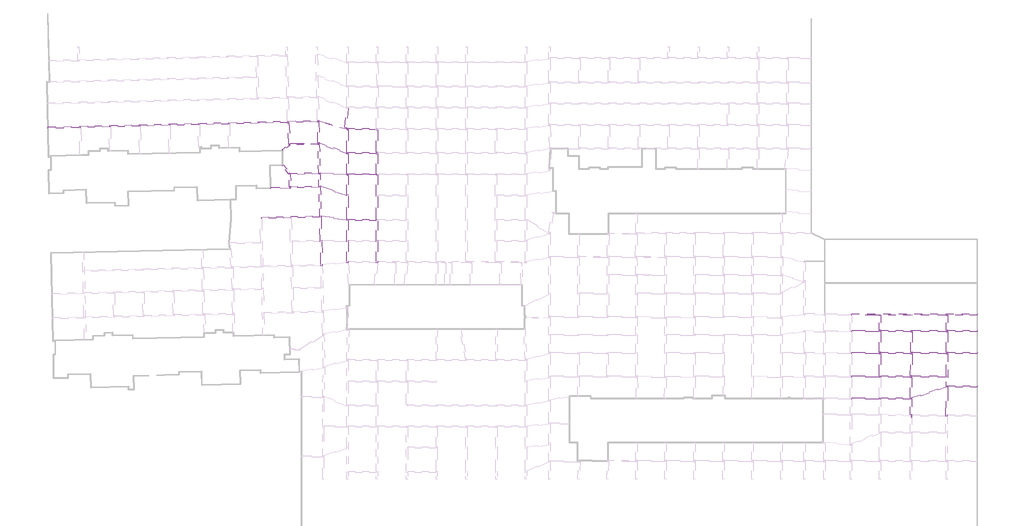
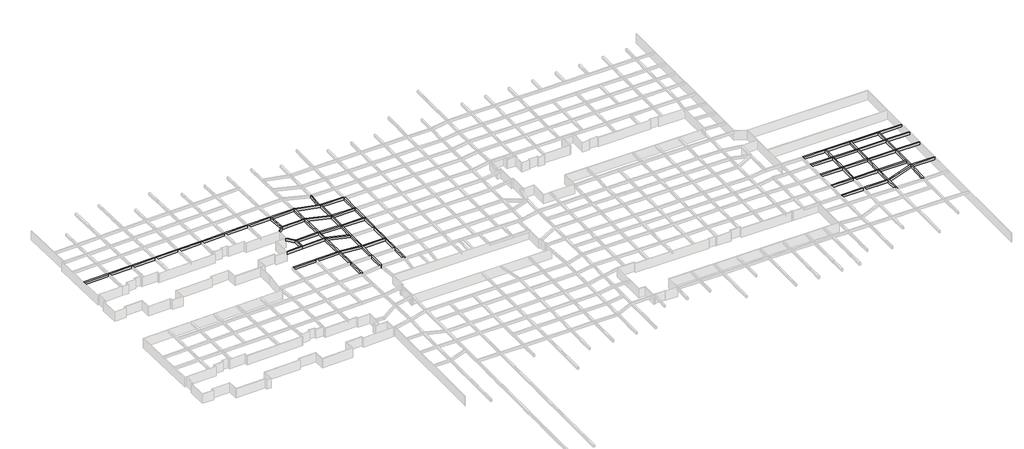
# One storey, part 16 of 20: 50 beams.
"""IFC4 building model written with IfcOpenShell, lengths in millimetres."""

import ifcopenshell
import ifcopenshell.guid

model = None  # the IFC model being written
_history = None  # IfcOwnerHistory: only IFC2X3 demands one
_inside = {}  # id of a spatial element -> (the spatial element, [elements in it])
_under = {}  # id of a project, library or spatial element -> (it, [spatial elements below it])
_declared = {}  # id of a project -> (the project, [libraries it declares])
_typed = {}  # id of a type object -> (the type object, [elements of that type])
_made_of = {}  # id of a material, layer set ... -> (it, [elements and type objects made of it])


def new_model(schema):
    """Start an empty IFC model of exactly this schema.

    Asked for "IFC4X3", IfcOpenShell would pick the latest addendum, in which some entities
    have other attributes; the version numbers below select the first issue.
    IFC2X3 requires an IfcOwnerHistory on every rooted entity: one is made here for all.
    """
    global model, _history
    if schema == "IFC4X3":
        model = ifcopenshell.file(schema_version=(4, 3, 0, 0))
    else:
        model = ifcopenshell.file(schema=schema)
    _inside.clear()
    _under.clear()
    _declared.clear()
    _typed.clear()
    _made_of.clear()
    _history = None
    if model.schema == "IFC2X3":
        org = make("IfcOrganization", Name="unknown")
        user = make(
            "IfcPersonAndOrganization",
            ThePerson=make("IfcPerson", FamilyName="unknown"),
            TheOrganization=org,
        )
        app = make(
            "IfcApplication",
            ApplicationDeveloper=org,
            Version="unknown",
            ApplicationFullName="unknown",
            ApplicationIdentifier="unknown",
        )
        _history = make(
            "IfcOwnerHistory",
            OwningUser=user,
            OwningApplication=app,
            ChangeAction="ADDED",
            CreationDate=0,
        )
    return model


def make(cls, **values):
    """One entity of the class cls with the attributes given. An attribute that is None is left unset."""
    return model.create_entity(
        cls, **{name: value for name, value in values.items() if value is not None}
    )


def rooted(cls, **values):
    """An entity with a GlobalId (a new one), such as an element, a storey or a relation."""
    return make(cls, GlobalId=ifcopenshell.guid.new(), OwnerHistory=_history, **values)


def si_unit(unit_type, name, prefix=None):
    """IfcSIUnit, for example si_unit("LENGTHUNIT", "METRE", prefix="MILLI")."""
    return make("IfcSIUnit", UnitType=unit_type, Prefix=prefix, Name=name)


def assignment(units):
    """IfcUnitAssignment: the units of a project."""
    return None if units is None else make("IfcUnitAssignment", Units=units)


def point(xyz):
    """IfcCartesianPoint."""
    return None if xyz is None else make("IfcCartesianPoint", Coordinates=xyz)


def direction(xyz):
    """IfcDirection."""
    return None if xyz is None else make("IfcDirection", DirectionRatios=xyz)


def frame(location, z_axis=None, x_axis=None):
    """IfcAxis2Placement3D, a coordinate frame: its origin and axes. An axis left out is left unset."""
    return make(
        "IfcAxis2Placement3D",
        Location=point(location),
        Axis=direction(z_axis),
        RefDirection=direction(x_axis),
    )


def origin():
    """The frame at (0, 0, 0) with its axes left unset."""
    return frame((0.0, 0.0, 0.0))


def place(relative_to, where):
    """IfcLocalPlacement: puts the frame where relative to a parent placement (None: the world)."""
    return make(
        "IfcLocalPlacement", PlacementRelTo=relative_to, RelativePlacement=where
    )


def context(
    kind, dimensions, precision=None, world=None, true_north=None, identifier=None
):
    """IfcGeometricRepresentationContext, for example the 3D "Model" context."""
    return make(
        "IfcGeometricRepresentationContext",
        ContextIdentifier=identifier,
        ContextType=kind,
        CoordinateSpaceDimension=dimensions,
        Precision=precision,
        WorldCoordinateSystem=world,
        TrueNorth=true_north,
    )


def project(units=None, contexts=None):
    """IfcProject with its units and contexts."""
    return rooted(
        "IfcProject",
        Name="project",
        RepresentationContexts=contexts,
        UnitsInContext=assignment(units),
    )


def spatial(cls, under=None, at=None, **own):
    """A site, building, storey or space (cls), placed at a placement, below another one or the project."""
    s = rooted(cls, ObjectPlacement=at, **own)
    if under is not None:
        _under.setdefault(under.id(), (under, []))[1].append(s)
    return s


def polyline(points):
    """IfcPolyline through the points."""
    return make("IfcPolyline", Points=[point(p) for p in points])


def outline(outer, holes=None, kind="AREA"):
    """IfcArbitraryClosedProfileDef: a profile drawn as a closed curve; with holes, ...WithVoids."""
    if holes is None:
        return make("IfcArbitraryClosedProfileDef", ProfileType=kind, OuterCurve=outer)
    return make(
        "IfcArbitraryProfileDefWithVoids",
        ProfileType=kind,
        OuterCurve=outer,
        InnerCurves=holes,
    )


def extrude(swept, where, along, depth):
    """IfcExtrudedAreaSolid: the profile swept, set in the frame where, extruded along a direction by depth."""
    return make(
        "IfcExtrudedAreaSolid",
        SweptArea=swept,
        Position=where,
        ExtrudedDirection=direction(along),
        Depth=depth,
    )


def faces_of(points, faces, orient=None, outer=None):
    """IfcFace entities. A face is a list of loops; a loop is a list of indices into points, from 0.

    orient and outer hold one flag for each loop. By default every Orientation is true, the
    first loop of a face is its IfcFaceOuterBound and the others are IfcFaceBound.
    """
    made = []
    for i, loops in enumerate(faces):
        bounds = []
        for j, loop in enumerate(loops):
            is_outer = j == 0 if outer is None else outer[i][j]
            bounds.append(
                make(
                    "IfcFaceOuterBound" if is_outer else "IfcFaceBound",
                    Bound=make("IfcPolyLoop", Polygon=[points[k] for k in loop]),
                    Orientation=True if orient is None else orient[i][j],
                )
            )
        made.append(make("IfcFace", Bounds=bounds))
    return made


def faceted_brep(points, faces, orient=None, outer=None, voids=None):
    """IfcFacetedBrep: a solid bounded by flat faces; with voids (closed shells), ...WithVoids."""
    shared = [point(p) for p in points]
    hull = make("IfcClosedShell", CfsFaces=faces_of(shared, faces, orient, outer))
    if voids is None:
        return make("IfcFacetedBrep", Outer=hull)
    return make(
        "IfcFacetedBrepWithVoids",
        Outer=hull,
        Voids=[
            make(cls, CfsFaces=faces_of(shared, fs, o, b)) for cls, fs, o, b in voids
        ],
    )


def shape(context_of_items, identifier, shape_type, items):
    """IfcShapeRepresentation: the items that make up one representation, for example the "Body"."""
    return make(
        "IfcShapeRepresentation",
        ContextOfItems=context_of_items,
        RepresentationIdentifier=identifier,
        RepresentationType=shape_type,
        Items=items,
    )


def made_of(thing, what):
    """Note that an element or type object is made of a material, layer set ...; save() writes the relation."""
    if what is not None:
        _made_of.setdefault(what.id(), (what, []))[1].append(thing)
    return thing


def element(
    cls,
    number,
    at=None,
    inside=None,
    cuts=None,
    type_object=None,
    material=None,
    context=None,
    identifier="Body",
    shape_type=None,
    held_by="IfcProductDefinitionShape",
    body=None,
    shapes=None,
    **own,
):
    """One element of the class cls, such as IfcWall. Its Tag is "e" and its number.

    at: its placement. inside: the storey or other place that contains it. cuts: it is an
    opening in that element (IfcRelVoidsElement). A single representation is given by context,
    identifier, shape_type and body (its items); several are given by shapes. held_by: the class
    of the entity that holds the representations. save() writes the other relations.
    """
    e = rooted(cls, Tag="e%d" % number, ObjectPlacement=at, **own)
    if body is not None:
        shapes = [shape(context, identifier, shape_type, body)]
    if shapes is not None:
        e.Representation = make(held_by, Representations=shapes)
    if inside is not None:
        _inside.setdefault(inside.id(), (inside, []))[1].append(e)
    if cuts is not None:
        rooted(
            "IfcRelVoidsElement", RelatingBuildingElement=cuts, RelatedOpeningElement=e
        )
    if type_object is not None:
        _typed.setdefault(type_object.id(), (type_object, []))[1].append(e)
    return made_of(e, material)


def aggregate(whole, parts):
    """IfcRelAggregates: a whole, such as a stair, and the parts it consists of."""
    return rooted("IfcRelAggregates", RelatingObject=whole, RelatedObjects=parts)


def save(model, path):
    """Write the relations noted so far, then the file.

    IfcRelAggregates (storeys below a building ...), IfcRelContainedInSpatialStructure (elements
    in a storey), IfcRelDefinesByType, IfcRelAssociatesMaterial and IfcRelDeclares: one each for
    every whole, place, type object, material and project.
    """
    for whole, parts in _under.values():
        aggregate(whole, parts)
    for where, things in _inside.values():
        rooted(
            "IfcRelContainedInSpatialStructure",
            RelatedElements=things,
            RelatingStructure=where,
        )
    for kind, things in _typed.values():
        rooted("IfcRelDefinesByType", RelatedObjects=things, RelatingType=kind)
    for what, things in _made_of.values():
        rooted("IfcRelAssociatesMaterial", RelatedObjects=things, RelatingMaterial=what)
    for by, libraries in _declared.values():
        rooted("IfcRelDeclares", RelatingContext=by, RelatedDefinitions=libraries)
    model.write(path)


model = new_model("IFC4")

# Units and contexts
model_context = context("Model", 3, world=origin())
ifc_project = project(units=[si_unit("LENGTHUNIT", "METRE", prefix="MILLI")], contexts=[model_context])

# Site, building, storey
site = spatial("IfcSite", under=ifc_project)
building = spatial("IfcBuilding", under=site)
storey = spatial("IfcBuildingStorey", under=building, Name="户型图", Elevation=0.0)

# Beams
placement = place(None, origin())
element("IfcBeam", 1, ObjectType="混凝土 - 矩形梁 : KL_beam", at=placement, inside=storey, context=model_context, shape_type="Brep", body=[
    faceted_brep([(-25852.2930768, 155817.7071887, 3300.0), (-25861.8581582, 156217.5928089, 3300.0), (-25861.8581582, 156217.5928089, 2500.0), (-25852.2930768, 155817.7071887, 2500.0), (-17401.6326758, 156019.8431266, 3300.0), (-17001.7470489, 156029.4082082, 3300.0), (-9404.088417, 156211.1407332, 3300.0), (-9004.2027939, 156220.7058147, 3300.0), (-1404.8339776, 156402.4792466, 3300.0), (-1004.9483311, 156412.0443286, 3300.0), (6573.7901577, 156593.3242925, 3300.0), (6973.6759029, 156602.8893769, 3300.0), (14546.0902706, 156784.0180707, 3300.0), (14945.9762348, 156793.5831603, 3300.0), (22591.0748231, 156976.4504274, 3300.0), (22990.9604712, 156986.0155095, 3300.0), (30570.1741778, 157167.3068404, 3300.0), (30970.0598259, 157176.8719225, 3300.0), (38519.8790772, 157357.4601514, 3300.0), (38920.1862756, 157367.0353168, 3300.0), (46582.3216226, 157550.3100954, 3300.0), (46982.2072428, 157559.8751768, 3300.0), (46973.8252673, 157910.2989037, 3300.0), (46972.6421614, 157959.760797, 3300.0), (46800.9210417, 157955.6533062, 3300.0), (46572.7215317, 157950.1948781, 3300.0), (38901.2269429, 157766.6962307, 3300.0), (38501.3413227, 157757.1311493, 3300.0), (30960.3453208, 157576.7539685, 3300.0), (30560.4596727, 157567.1888864, 3300.0), (22981.2459661, 157385.8975556, 3300.0), (22581.360318, 157376.3324735, 3300.0), (14936.9356889, 157193.4813271, 3300.0), (14537.0497247, 157183.9162375, 3300.0), (6964.4270838, 157002.7825619, 3300.0), (6564.5413385, 156993.2174775, 3300.0), (-1014.6584715, 156811.926479, 3300.0), (-1414.5441179, 156802.361397, 3300.0), (-9013.8162016, 156620.5902789, 3300.0), (-9413.7018247, 156611.0251974, 3300.0), (-17011.3853052, 156429.292078, 3300.0), (-17411.2709321, 156419.7269964, 3300.0), (46972.6421614, 157959.760797, 2500.0), (46800.9210417, 157955.6533062, 2500.0), (46572.7215317, 157950.1948781, 2500.0), (38901.2269429, 157766.6962307, 2500.0), (38501.3413227, 157757.1311493, 2500.0), (30960.3453208, 157576.7539685, 2500.0), (30560.4596727, 157567.1888864, 2500.0), (22981.2459661, 157385.8975556, 2500.0), (22581.360318, 157376.3324735, 2500.0), (14936.9356889, 157193.4813271, 2500.0), (14537.0497247, 157183.9162375, 2500.0), (6964.4270838, 157002.7825619, 2500.0), (6564.5413385, 156993.2174775, 2500.0), (-1014.6584715, 156811.926479, 2500.0), (-1414.5441179, 156802.361397, 2500.0), (-9013.8162016, 156620.5902789, 2500.0), (-9413.7018247, 156611.0251974, 2500.0), (-17011.3853052, 156429.292078, 2500.0), (-17411.2709321, 156419.7269964, 2500.0), (46973.8252673, 157910.2989037, 2500.0), (46982.2072428, 157559.8751768, 2500.0), (46582.3216226, 157550.3100954, 2500.0), (38920.1862756, 157367.0353168, 2500.0), (38519.8790772, 157357.4601514, 2500.0), (30970.0598259, 157176.8719225, 2500.0), (30570.1741778, 157167.3068404, 2500.0), (22990.9604712, 156986.0155095, 2500.0), (22591.0748231, 156976.4504274, 2500.0), (14945.9762348, 156793.5831603, 2500.0), (14546.0902706, 156784.0180707, 2500.0), (6973.6759029, 156602.8893769, 2500.0), (6573.7901577, 156593.3242925, 2500.0), (-1004.9483311, 156412.0443286, 2500.0), (-1404.8339776, 156402.4792466, 2500.0), (-9004.2027939, 156220.7058147, 2500.0), (-9404.088417, 156211.1407332, 2500.0), (-17001.7470489, 156029.4082082, 2500.0), (-17401.6326758, 156019.8431266, 2500.0)], [[[0, 1, 2, 3]], [[1, 0, 4, 5, 6, 7, 8, 9, 10, 11, 12, 13, 14, 15, 16, 17, 18, 19, 20, 21, 22, 23, 24, 25, 26, 27, 28, 29, 30, 31, 32, 33, 34, 35, 36, 37, 38, 39, 40, 41]], [[2, 1, 41, 40, 39, 38, 37, 36, 35, 34, 33, 32, 31, 30, 29, 28, 27, 26, 25, 24, 23, 42, 43, 44, 45, 46, 47, 48, 49, 50, 51, 52, 53, 54, 55, 56, 57, 58, 59, 60]], [[3, 2, 60, 59, 58, 57, 56, 55, 54, 53, 52, 51, 50, 49, 48, 47, 46, 45, 44, 43, 42, 61, 62, 63, 64, 65, 66, 67, 68, 69, 70, 71, 72, 73, 74, 75, 76, 77, 78, 79]], [[0, 3, 79, 78, 77, 76, 75, 74, 73, 72, 71, 70, 69, 68, 67, 66, 65, 64, 63, 62, 21, 20, 19, 18, 17, 16, 15, 14, 13, 12, 11, 10, 9, 8, 7, 6, 5, 4]], [[23, 22, 21, 62, 61, 42]]]),
])
element("IfcBeam", 2, ObjectType="混凝土 - 矩形梁 : KL_beam", at=placement, inside=storey, context=model_context, shape_type="Brep", body=[
    faceted_brep([(38953.8008449, 151152.0897698, 3300.0), (39202.1846675, 151368.0212907, 3300.0), (39331.7988752, 151480.7009037, 3300.0), (39311.5141423, 151770.7860982, 3300.0), (38920.1862756, 157367.0353168, 3300.0), (38519.8790772, 157357.4601514, 3300.0), (38918.8621266, 151651.7367193, 3300.0), (38953.8008449, 151152.0897698, 2500.0), (38519.8790772, 157357.4601514, 2500.0), (38918.8621266, 151651.7367193, 2500.0), (39331.7988752, 151480.7009037, 2500.0), (39202.1846675, 151368.0212907, 2500.0), (38920.1862756, 157367.0353168, 2500.0), (39311.5141423, 151770.7860982, 2500.0)], [[[0, 1, 2, 3, 4, 5, 6]], [[7, 0, 6, 5, 8, 9]], [[10, 11, 7, 9, 8, 12, 13]], [[2, 10, 13, 12, 4, 3]], [[5, 4, 12, 8]], [[2, 1, 0, 7, 11, 10]]]),
])
element("IfcBeam", 3, ObjectType="混凝土 - 矩形梁 : KL_beam", at=placement, inside=storey, context=model_context, shape_type="SweptSolid", body=[
    extrude(outline(polyline([(37366.5456098, 149772.2155356), (37104.111782, 150074.0904867), (38918.8621266, 151651.7367193), (38953.8008449, 151152.0897698), (37366.5456098, 149772.2155356)])), frame((0.0, 0.0, 2500.0), z_axis=(0.0, 0.0, 1.0), x_axis=(1.0, 0.0, 0.0)), (0.0, 0.0, 1.0), 800.0),
])
element("IfcBeam", 4, ObjectType="混凝土 - 矩形梁 : KL_beam", at=placement, inside=storey, context=model_context, shape_type="Brep", body=[
    faceted_brep([(39311.5141423, 151770.7860982, 3300.0), (39331.7988752, 151480.7009037, 3300.0), (39202.1846675, 151368.0212907, 3300.0), (46725.8596297, 151550.2158157, 3300.0), (46891.0426119, 151554.2159134, 3300.0), (47125.7239332, 151559.8989941, 3300.0), (47117.5771884, 151900.4884742, 3300.0), (47116.1588514, 151959.7846318, 3300.0), (46950.9573881, 151955.7840866, 3300.0), (46716.2760668, 151950.1010059, 3300.0), (39202.1846675, 151368.0212907, 2500.0), (46725.8596297, 151550.2158157, 2500.0), (46891.0426119, 151554.2159134, 2500.0), (47125.7239332, 151559.8989941, 2500.0), (39331.7988752, 151480.7009037, 2500.0), (39311.5141423, 151770.7860982, 2500.0), (46716.2760668, 151950.1010059, 2500.0), (46950.9573881, 151955.7840866, 2500.0), (47116.1588514, 151959.7846318, 2500.0), (47117.5771884, 151900.4884742, 2500.0)], [[[0, 1, 2, 3, 4, 5, 6, 7, 8, 9]], [[2, 10, 11, 12, 13, 5, 4, 3]], [[14, 15, 16, 17, 18, 19, 13, 12, 11, 10]], [[15, 0, 9, 8, 7, 18, 17, 16]], [[14, 1, 0, 15]], [[1, 14, 10, 2]], [[7, 6, 5, 13, 19, 18]]]),
])
element("IfcBeam", 5, ObjectType="混凝土 - 矩形梁 : KL_beam", at=placement, inside=storey, context=model_context, shape_type="Brep", body=[
    faceted_brep([(46982.2072428, 157559.8751768, 3300.0), (46582.3216226, 157550.3100954, 3300.0), (46716.2760668, 151950.1010059, 3300.0), (47116.1588514, 151959.7846318, 3300.0), (46983.7792263, 157494.1555485, 3300.0), (46982.2072428, 157559.8751768, 2500.0), (47116.1588514, 151959.7846318, 2500.0), (46983.7792263, 157494.1555485, 2500.0), (46582.3216226, 157550.3100954, 2500.0), (46716.2760668, 151950.1010059, 2500.0)], [[[0, 1, 2, 3, 4]], [[5, 0, 4, 3, 6, 7]], [[8, 5, 7, 6, 9]], [[1, 8, 9, 2]], [[1, 0, 5, 8]], [[3, 2, 9, 6]]]),
])
element("IfcBeam", 6, ObjectType="混凝土 - 矩形梁 : KL_beam", at=placement, inside=storey, context=model_context, shape_type="Brep", body=[
    faceted_brep([(54675.7946125, 155890.0, 3300.0), (54624.2053875, 155490.0, 3300.0), (54850.0, 155490.0, 3300.0), (62450.0, 155490.0, 3300.0), (62450.0, 155890.0, 3300.0), (54624.2053875, 155490.0, 2500.0), (54850.0, 155490.0, 2500.0), (62450.0, 155490.0, 2500.0), (54675.7946125, 155890.0, 2500.0), (62450.0, 155890.0, 2500.0)], [[[0, 1, 2, 3, 4]], [[1, 5, 6, 7, 3, 2]], [[5, 8, 9, 7, 6]], [[8, 0, 4, 9]], [[4, 3, 7, 9]], [[0, 8, 5, 1]]]),
])
element("IfcBeam", 7, ObjectType="混凝土 - 矩形梁 : KL_beam", at=placement, inside=storey, context=model_context, shape_type="SweptSolid", body=[
    extrude(outline(polyline([(54431.7382998, 161190.0), (54833.2662348, 161190.0), (54376.4460966, 155968.5219275), (53983.9261406, 156071.4835989), (54431.7382998, 161190.0)])), frame((0.0, 0.0, 2500.0), z_axis=(0.0, 0.0, 1.0), x_axis=(1.0, 0.0, 0.0)), (0.0, 0.0, 1.0), 800.0),
])
element("IfcBeam", 8, ObjectType="混凝土 - 矩形梁 : KL_beam", at=placement, inside=storey, context=model_context, shape_type="Brep", body=[
    faceted_brep([(46571.1845577, 158015.9153439, 3300.0), (46572.7565412, 157950.1957156, 3300.0), (46800.9210417, 157955.6533062, 3300.0), (46571.1845577, 158015.9153439, 2500.0), (46800.9210417, 157955.6533062, 2500.0), (46572.7565412, 157950.1957156, 2500.0)], [[[0, 1, 2]], [[3, 0, 2, 4]], [[5, 3, 4]], [[0, 3, 5, 1]], [[2, 1, 5, 4]]]),
    faceted_brep([(54624.2053875, 155490.0, 2500.0), (54624.2053875, 155490.0, 3300.0), (54450.0, 155535.6957094, 3300.0), (46983.7792263, 157494.1555485, 3300.0), (46983.7792263, 157494.1555485, 2500.0), (54450.0, 155535.6957094, 2500.0), (54675.7946125, 155890.0, 2500.0), (54675.7946125, 155890.0, 3300.0), (46973.8252673, 157910.2989037, 3300.0), (46973.8252673, 157910.2989037, 2500.0), (46982.2072428, 157559.8751768, 2500.0), (46982.2072428, 157559.8751768, 3300.0), (54376.4460966, 155968.5219275, 3300.0), (53983.9261406, 156071.4835989, 3300.0), (54376.4460966, 155968.5219275, 2500.0), (53983.9261406, 156071.4835989, 2500.0)], [[[0, 1, 2, 3, 4, 5]], [[1, 0, 6, 7]], [[8, 9, 10, 4, 3, 11]], [[1, 7, 12, 13, 8, 11, 3, 2]], [[7, 6, 14, 15, 9, 8, 13, 12]], [[6, 0, 5, 4, 10, 9, 15, 14]]]),
])
element("IfcBeam", 9, ObjectType="混凝土 - 矩形梁 : KL_beam", at=placement, inside=storey, context=model_context, shape_type="Brep", body=[
    faceted_brep([(54850.0, 149045.647444, 3300.0), (54850.0, 149390.0, 3300.0), (54850.0, 155490.0, 3300.0), (54624.2053875, 155490.0, 3300.0), (54450.0, 155535.6957094, 3300.0), (54450.0, 149467.0993538, 3300.0), (54450.0, 149045.647444, 3300.0), (54450.0, 149045.647444, 2500.0), (54450.0, 155535.6957094, 2500.0), (54450.0, 149467.0993538, 2500.0), (54850.0, 155490.0, 2500.0), (54850.0, 149390.0, 2500.0), (54850.0, 149045.647444, 2500.0), (54624.2053875, 155490.0, 2500.0)], [[[0, 1, 2, 3, 4, 5, 6]], [[7, 6, 5, 4, 8, 9]], [[10, 11, 12, 7, 9, 8, 13]], [[2, 1, 0, 12, 11, 10]], [[3, 2, 10, 13]], [[4, 3, 13, 8]], [[0, 6, 7, 12]]]),
])
element("IfcBeam", 10, ObjectType="混凝土 - 矩形梁 : KL_beam", at=placement, inside=storey, context=model_context, shape_type="Brep", body=[
    faceted_brep([(46891.0426119, 151554.2159134, 3300.0), (47127.7652717, 151475.6554758, 3300.0), (54450.0, 149045.647444, 3300.0), (54450.0, 149467.0993538, 3300.0), (47117.5771884, 151900.4884742, 3300.0), (47125.7239332, 151559.8989941, 3300.0), (46891.0426119, 151554.2159134, 2500.0), (47127.7652717, 151475.6554758, 2500.0), (54450.0, 149045.647444, 2500.0), (47125.7239332, 151559.8989941, 2500.0), (47117.5771884, 151900.4884742, 2500.0), (54450.0, 149467.0993538, 2500.0)], [[[0, 1, 2, 3, 4, 5]], [[2, 1, 0, 6, 7, 8]], [[8, 7, 6, 9, 10, 11]], [[10, 4, 3, 11]], [[5, 9, 6, 0]], [[9, 5, 4, 10]], [[3, 2, 8, 11]]]),
    faceted_brep([(46950.9573881, 151955.7840866, 3300.0), (46716.2575949, 151950.1005586, 3300.0), (46716.2575949, 151950.1005586, 2500.0), (46950.9573881, 151955.7840866, 2500.0), (46714.2347283, 152034.3445242, 3300.0), (46714.2347283, 152034.3445242, 2500.0)], [[[0, 1, 2, 3]], [[0, 4, 1]], [[5, 3, 2]], [[4, 0, 3, 5]], [[4, 5, 2, 1]]]),
])
element("IfcBeam", 11, ObjectType="混凝土 - 矩形梁 : KL_beam", at=placement, inside=storey, context=model_context, shape_type="Brep", body=[
    faceted_brep([(46917.5803344, 143565.8473025, 3300.0), (47111.0282939, 143558.9430301, 3300.0), (47318.0388271, 143551.5547014, 3300.0), (47308.4196656, 143952.1526975, 3300.0), (47127.7652717, 151475.6554758, 3300.0), (46891.0426119, 151554.2159134, 3300.0), (46725.8596297, 151550.2158157, 3300.0), (46908.2554629, 143954.1893463, 3300.0), (46725.8596297, 151550.2158157, 2500.0), (46908.2554629, 143954.1893463, 2500.0), (46917.5803344, 143565.8473025, 2500.0), (47318.0388271, 143551.5547014, 2500.0), (47111.0282939, 143558.9430301, 2500.0), (46891.0426119, 151554.2159134, 2500.0), (47127.7652717, 151475.6554758, 2500.0), (47308.4196656, 143952.1526975, 2500.0)], [[[0, 1, 2, 3, 4, 5, 6, 7]], [[6, 8, 9, 10, 0, 7]], [[11, 12, 10, 9, 8, 13, 14, 15]], [[2, 11, 15, 14, 4, 3]], [[8, 6, 5, 13]], [[5, 4, 14, 13]], [[2, 1, 0, 10, 12, 11]]]),
])
element("IfcBeam", 12, ObjectType="混凝土 - 矩形梁 : KL_beam", at=placement, inside=storey, context=model_context, shape_type="Brep", body=[
    faceted_brep([(54450.0, 143297.0107773, 3300.0), (54850.0, 143297.0107773, 3300.0), (54850.0, 143690.0, 3300.0), (54850.0, 148990.0, 3300.0), (54850.0, 149045.647444, 3300.0), (54450.0, 149045.647444, 3300.0), (54450.0, 143697.2654599, 3300.0), (54450.0, 143297.0107773, 2500.0), (54450.0, 149045.647444, 2500.0), (54450.0, 143697.2654599, 2500.0), (54850.0, 143297.0107773, 2500.0), (54850.0, 149045.647444, 2500.0), (54850.0, 148990.0, 2500.0), (54850.0, 143690.0, 2500.0)], [[[0, 1, 2, 3, 4, 5, 6]], [[7, 0, 6, 5, 8, 9]], [[10, 7, 9, 8, 11, 12, 13]], [[1, 10, 13, 12, 11, 4, 3, 2]], [[5, 4, 11, 8]], [[1, 0, 7, 10]]]),
])
element("IfcBeam", 13, ObjectType="混凝土 - 矩形梁 : KL_beam", at=placement, inside=storey, context=model_context, shape_type="Brep", body=[
    faceted_brep([(54850.0, 143282.7345401, 3300.0), (54850.0, 143290.0, 3300.0), (54850.0, 143297.0107773, 3300.0), (54450.0, 143297.0107773, 3300.0), (54646.4320766, 143290.0, 3300.0), (54850.0, 143282.7345401, 2500.0), (47318.0388271, 143551.5547014, 3300.0), (47318.0388271, 143551.5547014, 2500.0), (54450.0, 143297.0107773, 2500.0), (54646.4320766, 143290.0, 2500.0), (54850.0, 143297.0107773, 2500.0), (54850.0, 143290.0, 2500.0), (47308.4196656, 143952.1526975, 2500.0), (47308.4196656, 143952.1526975, 3300.0), (54450.0, 143697.2654599, 3300.0), (54450.0, 143697.2654599, 2500.0)], [[[0, 1, 2, 3, 4]], [[5, 0, 4, 3, 6, 7, 8, 9]], [[10, 11, 5, 9, 8]], [[12, 13, 14, 15]], [[0, 5, 11, 10, 2, 1]], [[6, 13, 12, 7]], [[3, 8, 15, 14]], [[8, 3, 2, 10]], [[13, 6, 3, 14]], [[7, 12, 15, 8]]]),
])
element("IfcBeam", 14, ObjectType="混凝土 - 矩形梁 : KL_beam", at=placement, inside=storey, context=model_context, shape_type="Brep", body=[
    faceted_brep([(54850.0, 149390.0, 3300.0), (54850.0, 149045.647444, 3300.0), (54850.0, 148990.0, 3300.0), (62450.0, 148990.0, 3300.0), (62850.0, 148990.0, 3300.0), (62850.0, 149390.0, 3300.0), (62450.0, 149390.0, 3300.0), (62850.0, 148990.0, 2500.0), (54850.0, 148990.0, 2500.0), (62450.0, 148990.0, 2500.0), (54850.0, 149045.647444, 2500.0), (54850.0, 149390.0, 2500.0), (62450.0, 149390.0, 2500.0), (62850.0, 149390.0, 2500.0)], [[[0, 1, 2, 3, 4, 5, 6]], [[7, 4, 3, 2, 8, 9]], [[8, 10, 11, 12, 13, 7, 9]], [[11, 0, 6, 5, 13, 12]], [[0, 11, 10, 8, 2, 1]], [[5, 4, 7, 13]]]),
])
element("IfcBeam", 15, ObjectType="混凝土 - 矩形梁 : KL_beam", at=placement, inside=storey, context=model_context, shape_type="Brep", body=[
    faceted_brep([(62450.0, 143290.0, 3300.0), (62850.0, 143290.0, 3300.0), (62850.0, 143690.0, 3300.0), (62850.0, 148990.0, 3300.0), (62450.0, 148990.0, 3300.0), (62450.0, 143690.0, 3300.0), (62450.0, 143290.0, 2500.0), (62450.0, 148990.0, 2500.0), (62450.0, 143690.0, 2500.0), (62850.0, 143290.0, 2500.0), (62850.0, 148990.0, 2500.0), (62850.0, 143690.0, 2500.0)], [[[0, 1, 2, 3, 4, 5]], [[6, 0, 5, 4, 7, 8]], [[9, 6, 8, 7, 10, 11]], [[1, 9, 11, 10, 3, 2]], [[4, 3, 10, 7]], [[1, 0, 6, 9]]]),
])
element("IfcBeam", 16, ObjectType="混凝土 - 矩形梁 : KL_beam", at=placement, inside=storey, context=model_context, shape_type="Brep", body=[
    faceted_brep([(54850.0, 143690.0, 3300.0), (54850.0, 143297.0107773, 3300.0), (54850.0, 143290.0, 3300.0), (62450.0, 143290.0, 3300.0), (62450.0, 143690.0, 3300.0), (54850.0, 143290.0, 2500.0), (62450.0, 143290.0, 2500.0), (54850.0, 143297.0107773, 2500.0), (54850.0, 143690.0, 2500.0), (62450.0, 143690.0, 2500.0)], [[[0, 1, 2, 3, 4]], [[2, 5, 6, 3]], [[5, 7, 8, 9, 6]], [[8, 0, 4, 9]], [[0, 8, 7, 5, 2, 1]], [[4, 3, 6, 9]]]),
    faceted_brep([(54450.0, 143290.0, 2500.0), (54450.0, 143290.0, 3300.0), (54450.0, 143297.0107773, 3300.0), (54450.0, 143297.0107773, 2500.0), (54646.4320766, 143290.0, 3300.0), (54646.4320766, 143290.0, 2500.0)], [[[0, 1, 2, 3]], [[2, 4, 5, 3]], [[1, 4, 2]], [[1, 0, 5, 4]], [[5, 0, 3]]]),
])
element("IfcBeam", 17, ObjectType="混凝土 - 矩形梁 : KL_beam", at=placement, inside=storey, context=model_context, shape_type="SweptSolid", body=[
    extrude(outline(polyline([(62450.0, 155490.0), (62850.0, 155490.0), (62850.0, 149390.0), (62450.0, 149390.0), (62450.0, 155490.0)])), frame((0.0, 0.0, 2500.0), z_axis=(0.0, 0.0, 1.0), x_axis=(1.0, 0.0, 0.0)), (0.0, 0.0, 1.0), 800.0),
])
element("IfcBeam", 18, ObjectType="混凝土 - 矩形梁 : KL_beam", at=placement, inside=storey, context=model_context, shape_type="Brep", body=[
    faceted_brep([(62450.0, 119690.0, 3300.0), (62832.0174047, 119690.0, 3300.0), (62850.0, 119690.0, 3300.0), (62850.0, 120090.0, 3300.0), (62850.0, 125365.1975441, 3300.0), (62850.0, 125765.1975441, 3300.0), (62850.0, 131060.9938217, 3300.0), (62850.0, 131460.9938217, 3300.0), (62850.0, 137602.152967, 3300.0), (62850.0, 138002.152967, 3300.0), (62850.0, 143290.0, 3300.0), (62450.0, 143290.0, 3300.0), (62450.0, 138002.152967, 3300.0), (62450.0, 137602.152967, 3300.0), (62450.0, 131460.9938217, 3300.0), (62450.0, 131060.9938217, 3300.0), (62450.0, 125765.1975441, 3300.0), (62450.0, 125365.1975441, 3300.0), (62450.0, 120090.0, 3300.0), (62450.0, 119690.0, 2500.0), (62450.0, 143290.0, 2500.0), (62450.0, 138002.152967, 2500.0), (62450.0, 137602.152967, 2500.0), (62450.0, 131460.9938217, 2500.0), (62450.0, 131060.9938217, 2500.0), (62450.0, 125765.1975441, 2500.0), (62450.0, 125365.1975441, 2500.0), (62450.0, 120090.0, 2500.0), (62850.0, 119690.0, 2500.0), (62832.0174047, 119690.0, 2500.0), (62850.0, 143290.0, 2500.0), (62850.0, 138002.152967, 2500.0), (62850.0, 137602.152967, 2500.0), (62850.0, 131460.9938217, 2500.0), (62850.0, 131060.9938217, 2500.0), (62850.0, 125765.1975441, 2500.0), (62850.0, 125365.1975441, 2500.0), (62850.0, 120090.0, 2500.0)], [[[0, 1, 2, 3, 4, 5, 6, 7, 8, 9, 10, 11, 12, 13, 14, 15, 16, 17, 18]], [[19, 0, 18, 17, 16, 15, 14, 13, 12, 11, 20, 21, 22, 23, 24, 25, 26, 27]], [[28, 29, 19, 27, 26, 25, 24, 23, 22, 21, 20, 30, 31, 32, 33, 34, 35, 36, 37]], [[2, 28, 37, 36, 35, 34, 33, 32, 31, 30, 10, 9, 8, 7, 6, 5, 4, 3]], [[11, 10, 30, 20]], [[2, 1, 0, 19, 29, 28]]]),
])
element("IfcBeam", 19, ObjectType="混凝土 - 矩形梁 : KL_beam", at=placement, inside=storey, context=model_context, shape_type="Brep", body=[
    faceted_brep([(54450.0, 119664.8886593, 3300.0), (54467.8976834, 119667.0104964, 3300.0), (54661.8140065, 119690.0, 3300.0), (54850.0, 119712.3101516, 3300.0), (54850.0, 120090.0, 3300.0), (54850.0, 125365.1975441, 3300.0), (54850.0, 125765.1975441, 3300.0), (54850.0, 131060.9938217, 3300.0), (54850.0, 131460.9938217, 3300.0), (54850.0, 137602.152967, 3300.0), (54850.0, 138002.152967, 3300.0), (54850.0, 143282.7345401, 3300.0), (54646.4320766, 143290.0, 3300.0), (54450.0, 143290.0, 3300.0), (54450.0, 138077.4293511, 3300.0), (54450.0, 137656.8444614, 3300.0), (54450.0, 131487.0526989, 3300.0), (54450.0, 131084.0487688, 3300.0), (54450.0, 125765.1975441, 3300.0), (54450.0, 125365.1975441, 3300.0), (54450.0, 120067.6898484, 3300.0), (54450.0, 119664.8886593, 2500.0), (54450.0, 143290.0, 2500.0), (54450.0, 138077.4293511, 2500.0), (54450.0, 137656.8444614, 2500.0), (54450.0, 131487.0526989, 2500.0), (54450.0, 131084.0487688, 2500.0), (54450.0, 125765.1975441, 2500.0), (54450.0, 125365.1975441, 2500.0), (54450.0, 120067.6898484, 2500.0), (54850.0, 119712.3101516, 2500.0), (54661.8140065, 119690.0, 2500.0), (54467.8976834, 119667.0104964, 2500.0), (54646.4320766, 143290.0, 2500.0), (54850.0, 143282.7345401, 2500.0), (54850.0, 138002.152967, 2500.0), (54850.0, 137602.152967, 2500.0), (54850.0, 131460.9938217, 2500.0), (54850.0, 131060.9938217, 2500.0), (54850.0, 125765.1975441, 2500.0), (54850.0, 125365.1975441, 2500.0), (54850.0, 120090.0, 2500.0)], [[[0, 1, 2, 3, 4, 5, 6, 7, 8, 9, 10, 11, 12, 13, 14, 15, 16, 17, 18, 19, 20]], [[21, 0, 20, 19, 18, 17, 16, 15, 14, 13, 22, 23, 24, 25, 26, 27, 28, 29]], [[30, 31, 32, 21, 29, 28, 27, 26, 25, 24, 23, 22, 33, 34, 35, 36, 37, 38, 39, 40, 41]], [[34, 11, 10, 9, 8, 7, 6, 5, 4, 3, 30, 41, 40, 39, 38, 37, 36, 35]], [[11, 34, 33, 12]], [[13, 12, 33, 22]], [[3, 2, 1, 0, 21, 32, 31, 30]]]),
])
element("IfcBeam", 20, ObjectType="混凝土 - 矩形梁 : KL_beam", at=placement, inside=storey, context=model_context, shape_type="Brep", body=[
    faceted_brep([(47912.3274647, 118889.8231887, 3300.0), (47902.648865, 119291.4769437, 3300.0), (47756.2911881, 125365.1975441, 3300.0), (47746.6524387, 125765.1975441, 3300.0), (47598.2122045, 131925.3425246, 3300.0), (47588.472252, 132329.5423706, 3300.0), (47404.9412965, 139945.9227953, 3300.0), (47394.7265387, 140369.826661, 3300.0), (47318.0568561, 143551.5540579, 3300.0), (46917.5963324, 143565.8467315, 3300.0), (46994.9485294, 140355.7955585, 3300.0), (47004.5844815, 139955.9116398, 3300.0), (47187.6808955, 132357.5643226, 3300.0), (47197.3168477, 131957.6804039, 3300.0), (47345.6819506, 125800.6533117, 3300.0), (47355.3179028, 125400.7693931, 3300.0), (47503.2400646, 119262.1239832, 3300.0), (47512.443546, 118880.1872365, 3300.0), (46917.5963324, 143565.8467315, 2500.0), (46994.9485294, 140355.7955585, 2500.0), (47004.5844815, 139955.9116398, 2500.0), (47187.6808955, 132357.5643226, 2500.0), (47197.3168477, 131957.6804039, 2500.0), (47345.6819506, 125800.6533117, 2500.0), (47355.3179028, 125400.7693931, 2500.0), (47503.2400646, 119262.1239832, 2500.0), (47512.443546, 118880.1872365, 2500.0), (47318.0568561, 143551.5540579, 2500.0), (47394.7265387, 140369.826661, 2500.0), (47404.9412965, 139945.9227953, 2500.0), (47588.472252, 132329.5423706, 2500.0), (47598.2122045, 131925.3425246, 2500.0), (47746.6524387, 125765.1975441, 2500.0), (47756.2911881, 125365.1975441, 2500.0), (47902.648865, 119291.4769437, 2500.0), (47912.3274647, 118889.8231887, 2500.0)], [[[0, 1, 2, 3, 4, 5, 6, 7, 8, 9, 10, 11, 12, 13, 14, 15, 16, 17]], [[17, 16, 15, 14, 13, 12, 11, 10, 9, 18, 19, 20, 21, 22, 23, 24, 25, 26]], [[26, 25, 24, 23, 22, 21, 20, 19, 18, 27, 28, 29, 30, 31, 32, 33, 34, 35]], [[8, 7, 6, 5, 4, 3, 2, 1, 0, 35, 34, 33, 32, 31, 30, 29, 28, 27]], [[9, 8, 27, 18]], [[0, 17, 26, 35]]]),
])
element("IfcBeam", 21, ObjectType="混凝土 - 矩形梁 : KL_beam", at=placement, inside=storey, context=model_context, shape_type="SweptSolid", body=[
    extrude(outline(polyline([(54450.0, 138077.4293511), (54450.0, 137656.8444614), (47404.9412965, 139945.9227953), (47394.7265387, 140369.826661), (54450.0, 138077.4293511)])), frame((0.0, 0.0, 2500.0), z_axis=(0.0, 0.0, 1.0), x_axis=(1.0, 0.0, 0.0)), (0.0, 0.0, 1.0), 800.0),
])
element("IfcBeam", 22, ObjectType="混凝土 - 矩形梁 : KL_beam", at=placement, inside=storey, context=model_context, shape_type="SweptSolid", body=[
    extrude(outline(polyline([(54450.0, 131487.0526989), (54450.0, 131084.0487688), (47598.2122045, 131925.3425246), (47588.472252, 132329.5423706), (54450.0, 131487.0526989)])), frame((0.0, 0.0, 2500.0), z_axis=(0.0, 0.0, 1.0), x_axis=(1.0, 0.0, 0.0)), (0.0, 0.0, 1.0), 800.0),
])
element("IfcBeam", 23, ObjectType="混凝土 - 矩形梁 : KL_beam", at=placement, inside=storey, context=model_context, shape_type="SweptSolid", body=[
    extrude(outline(polyline([(62450.0, 131460.9938217), (62450.0, 131060.9938217), (54850.0, 131060.9938217), (54850.0, 131460.9938217), (62450.0, 131460.9938217)])), frame((0.0, 0.0, 2500.0), z_axis=(0.0, 0.0, 1.0), x_axis=(1.0, 0.0, 0.0)), (0.0, 0.0, 1.0), 800.0),
])
element("IfcBeam", 24, ObjectType="混凝土 - 矩形梁 : KL_beam", at=placement, inside=storey, context=model_context, shape_type="Brep", body=[
    faceted_brep([(197950.0, 95263.9194786, 3300.0), (197950.0, 95663.9194786, 3300.0), (197550.0, 95663.9194786, 3300.0), (190150.0341333, 95663.9194786, 3300.0), (190150.0341333, 95263.9194786, 3300.0), (197550.0, 95263.9194786, 3300.0), (197950.0, 95263.9194786, 2500.0), (190150.0341333, 95263.9194786, 2500.0), (197550.0, 95263.9194786, 2500.0), (197950.0, 95663.9194786, 2500.0), (190150.0341333, 95663.9194786, 2500.0), (197550.0, 95663.9194786, 2500.0)], [[[0, 1, 2, 3, 4, 5]], [[6, 0, 5, 4, 7, 8]], [[9, 6, 8, 7, 10, 11]], [[1, 9, 11, 10, 3, 2]], [[4, 3, 10, 7]], [[1, 0, 6, 9]]]),
])
element("IfcBeam", 25, ObjectType="混凝土 - 矩形梁 : KL_beam", at=placement, inside=storey, context=model_context, shape_type="Brep", body=[
    faceted_brep([(197950.0, 101550.0, 3300.0), (197550.0, 101550.0, 3300.0), (197550.0, 101150.0, 3300.0), (197550.0, 95663.9194786, 3300.0), (197950.0, 95663.9194786, 3300.0), (197950.0, 101150.0, 3300.0), (197550.0, 101550.0, 2500.0), (197550.0, 101150.0, 2500.0), (197550.0, 95663.9194786, 2500.0), (197950.0, 101550.0, 2500.0), (197950.0, 101150.0, 2500.0), (197950.0, 95663.9194786, 2500.0)], [[[0, 1, 2, 3, 4, 5]], [[1, 6, 7, 8, 3, 2]], [[6, 9, 10, 11, 8, 7]], [[9, 0, 5, 4, 11, 10]], [[4, 3, 8, 11]], [[1, 0, 9, 6]]]),
])
element("IfcBeam", 26, ObjectType="混凝土 - 矩形梁 : KL_beam", at=placement, inside=storey, context=model_context, shape_type="Brep", body=[
    faceted_brep([(197550.0, 88891.7476257, 3300.0), (197562.0, 88891.7476257, 3300.0), (197950.0, 88891.7476257, 3300.0), (197950.0, 89291.7476257, 3300.0), (197950.0, 95263.9194786, 3300.0), (197550.0, 95263.9194786, 3300.0), (197550.0, 89291.7476257, 3300.0), (197550.0, 88891.7476257, 2500.0), (197550.0, 95263.9194786, 2500.0), (197550.0, 89291.7476257, 2500.0), (197950.0, 88891.7476257, 2500.0), (197562.0, 88891.7476257, 2500.0), (197950.0, 95263.9194786, 2500.0), (197950.0, 89291.7476257, 2500.0)], [[[0, 1, 2, 3, 4, 5, 6]], [[7, 0, 6, 5, 8, 9]], [[10, 11, 7, 9, 8, 12, 13]], [[2, 10, 13, 12, 4, 3]], [[5, 4, 12, 8]], [[2, 1, 0, 7, 11, 10]]]),
])
element("IfcBeam", 27, ObjectType="混凝土 - 矩形梁 : KL_beam", at=placement, inside=storey, context=model_context, shape_type="SweptSolid", body=[
    extrude(outline(polyline([(190150.0341333, 88891.7476257), (190150.0341333, 89291.7476257), (197550.0, 89291.7476257), (197550.0, 88891.7476257), (190150.0341333, 88891.7476257)])), frame((0.0, 0.0, 2500.0), z_axis=(0.0, 0.0, 1.0), x_axis=(1.0, 0.0, 0.0)), (0.0, 0.0, 1.0), 800.0),
])
element("IfcBeam", 28, ObjectType="混凝土 - 矩形梁 : KL_beam", at=placement, inside=storey, context=model_context, shape_type="Brep", body=[
    faceted_brep([(223897.5170667, 106050.0, 3300.0), (223897.5170667, 105650.0, 3300.0), (223897.5170667, 105650.0, 2500.0), (223897.5170667, 106050.0, 2500.0), (190150.0341333, 106050.0, 3300.0), (190150.0341333, 105650.0, 3300.0), (197550.0, 105650.0, 3300.0), (197950.0, 105650.0, 3300.0), (206038.0201399, 105650.0, 3300.0), (206438.0201399, 105650.0, 3300.0), (215638.0201399, 105650.0, 3300.0), (216038.0201399, 105650.0, 3300.0), (190150.0341333, 105650.0, 2500.0), (197550.0, 105650.0, 2500.0), (197950.0, 105650.0, 2500.0), (206038.0201399, 105650.0, 2500.0), (206438.0201399, 105650.0, 2500.0), (215638.0201399, 105650.0, 2500.0), (216038.0201399, 105650.0, 2500.0), (190150.0341333, 106050.0, 2500.0)], [[[0, 1, 2, 3]], [[1, 0, 4, 5, 6, 7, 8, 9, 10, 11]], [[2, 1, 11, 10, 9, 8, 7, 6, 5, 12, 13, 14, 15, 16, 17, 18]], [[3, 2, 18, 17, 16, 15, 14, 13, 12, 19]], [[0, 3, 19, 4]], [[5, 4, 19, 12]]]),
])
element("IfcBeam", 29, ObjectType="混凝土 - 矩形梁 : KL_beam", at=placement, inside=storey, context=model_context, shape_type="Brep", body=[
    faceted_brep([(223850.0, 101550.0, 3300.0), (223850.0, 101150.0, 3300.0), (223850.0, 101150.0, 2500.0), (223850.0, 101550.0, 2500.0), (216038.0201399, 101550.0, 3300.0), (215638.0201399, 101550.0, 3300.0), (206438.0201399, 101550.0, 3300.0), (206038.0201399, 101550.0, 3300.0), (197950.0, 101550.0, 3300.0), (197950.0, 101150.0, 3300.0), (206038.0201399, 101150.0, 3300.0), (206438.0201399, 101150.0, 3300.0), (215638.0201399, 101150.0, 3300.0), (216038.0201399, 101150.0, 3300.0), (197950.0, 101150.0, 2500.0), (206038.0201399, 101150.0, 2500.0), (206438.0201399, 101150.0, 2500.0), (215638.0201399, 101150.0, 2500.0), (216038.0201399, 101150.0, 2500.0), (197950.0, 101550.0, 2500.0), (206038.0201399, 101550.0, 2500.0), (206438.0201399, 101550.0, 2500.0), (215638.0201399, 101550.0, 2500.0), (216038.0201399, 101550.0, 2500.0)], [[[0, 1, 2, 3]], [[1, 0, 4, 5, 6, 7, 8, 9, 10, 11, 12, 13]], [[2, 1, 13, 12, 11, 10, 9, 14, 15, 16, 17, 18]], [[3, 2, 18, 17, 16, 15, 14, 19, 20, 21, 22, 23]], [[0, 3, 23, 22, 21, 20, 19, 8, 7, 6, 5, 4]], [[9, 8, 19, 14]]]),
])
element("IfcBeam", 30, ObjectType="混凝土 - 矩形梁 : KL_beam", at=placement, inside=storey, context=model_context, shape_type="Brep", body=[
    faceted_brep([(223850.0, 95663.9194786, 3300.0), (223850.0, 95263.9194786, 3300.0), (223850.0, 95263.9194786, 2500.0), (223850.0, 95663.9194786, 2500.0), (216038.0201399, 95663.9194786, 3300.0), (215638.0201399, 95663.9194786, 3300.0), (206438.0201399, 95663.9194786, 3300.0), (206038.0201399, 95663.9194786, 3300.0), (197950.0, 95663.9194786, 3300.0), (197950.0, 95263.9194786, 3300.0), (206034.4986613, 95263.9194786, 3300.0), (206434.5595925, 95263.9194786, 3300.0), (215638.0201399, 95263.9194786, 3300.0), (216038.0201399, 95263.9194786, 3300.0), (197950.0, 95263.9194786, 2500.0), (206034.4986613, 95263.9194786, 2500.0), (206434.5595925, 95263.9194786, 2500.0), (215638.0201399, 95263.9194786, 2500.0), (216038.0201399, 95263.9194786, 2500.0), (197950.0, 95663.9194786, 2500.0), (206038.0201399, 95663.9194786, 2500.0), (206438.0201399, 95663.9194786, 2500.0), (215638.0201399, 95663.9194786, 2500.0), (216038.0201399, 95663.9194786, 2500.0)], [[[0, 1, 2, 3]], [[1, 0, 4, 5, 6, 7, 8, 9, 10, 11, 12, 13]], [[2, 1, 13, 12, 11, 10, 9, 14, 15, 16, 17, 18]], [[3, 2, 18, 17, 16, 15, 14, 19, 20, 21, 22, 23]], [[0, 3, 23, 22, 21, 20, 19, 8, 7, 6, 5, 4]], [[9, 8, 19, 14]]]),
])
element("IfcBeam", 31, ObjectType="混凝土 - 矩形梁 : KL_beam", at=placement, inside=storey, context=model_context, shape_type="SweptSolid", body=[
    extrude(outline(polyline([(206034.4986613, 95263.9194786), (206434.5595925, 95263.9194786), (206330.3149451, 89291.7476257), (205930.2540139, 89291.7476257), (206034.4986613, 95263.9194786)])), frame((0.0, 0.0, 2500.0), z_axis=(0.0, 0.0, 1.0), x_axis=(1.0, 0.0, 0.0)), (0.0, 0.0, 1.0), 800.0),
])
element("IfcBeam", 32, ObjectType="混凝土 - 矩形梁 : KL_beam", at=placement, inside=storey, context=model_context, shape_type="SweptSolid", body=[
    extrude(outline(polyline([(206438.0201399, 95663.9194786), (206038.0201399, 95663.9194786), (206038.0201399, 101150.0), (206438.0201399, 101150.0), (206438.0201399, 95663.9194786)])), frame((0.0, 0.0, 2500.0), z_axis=(0.0, 0.0, 1.0), x_axis=(1.0, 0.0, 0.0)), (0.0, 0.0, 1.0), 800.0),
    extrude(outline(polyline([(206038.0201399, 105650.0), (206438.0201399, 105650.0), (206438.0201399, 101550.0), (206038.0201399, 101550.0), (206038.0201399, 105650.0)])), frame((0.0, 0.0, 2500.0), z_axis=(0.0, 0.0, 1.0), x_axis=(1.0, 0.0, 0.0)), (0.0, 0.0, 1.0), 800.0),
])
element("IfcBeam", 33, ObjectType="混凝土 - 矩形梁 : KL_beam", at=placement, inside=storey, context=model_context, shape_type="SweptSolid", body=[
    extrude(outline(polyline([(197950.0, 101550.0), (197550.0, 101550.0), (197550.0, 105650.0), (197950.0, 105650.0), (197950.0, 101550.0)])), frame((0.0, 0.0, 2500.0), z_axis=(0.0, 0.0, 1.0), x_axis=(1.0, 0.0, 0.0)), (0.0, 0.0, 1.0), 800.0),
])
element("IfcBeam", 34, ObjectType="混凝土 - 矩形梁 : KL_beam", at=placement, inside=storey, context=model_context, shape_type="SweptSolid", body=[
    extrude(outline(polyline([(197550.0, 101550.0), (197550.0, 101150.0), (190150.0341333, 101150.0), (190150.0341333, 101550.0), (197550.0, 101550.0)])), frame((0.0, 0.0, 2500.0), z_axis=(0.0, 0.0, 1.0), x_axis=(1.0, 0.0, 0.0)), (0.0, 0.0, 1.0), 800.0),
])
element("IfcBeam", 35, ObjectType="混凝土 - 矩形梁 : KL_beam", at=placement, inside=storey, context=model_context, shape_type="SweptSolid", body=[
    extrude(outline(polyline([(215638.0201399, 105650.0), (216038.0201399, 105650.0), (216038.0201399, 101550.0), (215638.0201399, 101550.0), (215638.0201399, 105650.0)])), frame((0.0, 0.0, 2500.0), z_axis=(0.0, 0.0, 1.0), x_axis=(1.0, 0.0, 0.0)), (0.0, 0.0, 1.0), 800.0),
])
element("IfcBeam", 36, ObjectType="混凝土 - 矩形梁 : KL_beam", at=placement, inside=storey, context=model_context, shape_type="SweptSolid", body=[
    extrude(outline(polyline([(215638.0201399, 101150.0), (216038.0201399, 101150.0), (216038.0201399, 95663.9194786), (215638.0201399, 95663.9194786), (215638.0201399, 101150.0)])), frame((0.0, 0.0, 2500.0), z_axis=(0.0, 0.0, 1.0), x_axis=(1.0, 0.0, 0.0)), (0.0, 0.0, 1.0), 800.0),
])
element("IfcBeam", 37, ObjectType="混凝土 - 矩形梁 : KL_beam", at=placement, inside=storey, context=model_context, shape_type="Brep", body=[
    faceted_brep([(215638.0201399, 86468.2056897, 3300.0), (216038.0201399, 86463.3089468, 3300.0), (216038.0201399, 86665.7573183, 3300.0), (216038.0201399, 95263.9194786, 3300.0), (215638.0201399, 95263.9194786, 3300.0), (215638.0201399, 89291.7476257, 3300.0), (215638.0201399, 88891.7476257, 3300.0), (215638.0201399, 86609.7869731, 3300.0), (215638.0201399, 86468.2056897, 2500.0), (215638.0201399, 95263.9194786, 2500.0), (215638.0201399, 89291.7476257, 2500.0), (215638.0201399, 88891.7476257, 2500.0), (215638.0201399, 86609.7869731, 2500.0), (216038.0201399, 86463.3089468, 2500.0), (216038.0201399, 95263.9194786, 2500.0), (216038.0201399, 86665.7573183, 2500.0)], [[[0, 1, 2, 3, 4, 5, 6, 7]], [[8, 0, 7, 6, 5, 4, 9, 10, 11, 12]], [[13, 8, 12, 11, 10, 9, 14, 15]], [[1, 13, 15, 14, 3, 2]], [[4, 3, 14, 9]], [[1, 0, 8, 13]]]),
])
element("IfcBeam", 38, ObjectType="混凝土 - 矩形梁 : KL_beam", at=placement, inside=storey, context=model_context, shape_type="Brep", body=[
    faceted_brep([(197950.0, 89291.7476257, 3300.0), (197950.0, 88891.7476257, 3300.0), (197962.0, 88891.7476257, 3300.0), (205926.7934665, 88891.7476257, 3300.0), (206326.7934665, 88891.7476257, 3300.0), (215638.0201399, 88891.7476257, 3300.0), (215638.0201399, 89291.7476257, 3300.0), (206330.3149451, 89291.7476257, 3300.0), (205930.2540139, 89291.7476257, 3300.0), (197950.0, 88891.7476257, 2500.0), (197962.0, 88891.7476257, 2500.0), (205926.7934665, 88891.7476257, 2500.0), (206326.7934665, 88891.7476257, 2500.0), (215638.0201399, 88891.7476257, 2500.0), (197950.0, 89291.7476257, 2500.0), (205930.2540139, 89291.7476257, 2500.0), (206330.3149451, 89291.7476257, 2500.0), (215638.0201399, 89291.7476257, 2500.0)], [[[0, 1, 2, 3, 4, 5, 6, 7, 8]], [[1, 9, 10, 11, 12, 13, 5, 4, 3, 2]], [[9, 14, 15, 16, 17, 13, 12, 11, 10]], [[14, 0, 8, 7, 6, 17, 16, 15]], [[1, 0, 14, 9]], [[6, 5, 13, 17]]]),
])
element("IfcBeam", 39, ObjectType="混凝土 - 矩形梁 : KL_beam", at=placement, inside=storey, context=model_context, shape_type="Brep", body=[
    faceted_brep([(215842.1624774, 78465.0, 3300.0), (215851.957431, 78865.0, 3300.0), (216033.1826173, 86265.7573183, 3300.0), (216038.0201399, 86463.3089468, 3300.0), (215638.0201399, 86468.2056897, 3300.0), (215631.1029221, 86185.72481, 3300.0), (215451.86201, 78866.0, 3300.0), (215442.2823499, 78474.7920182, 3300.0), (215638.0201399, 86468.2056897, 2500.0), (215631.1029221, 86185.72481, 2500.0), (215451.86201, 78866.0, 2500.0), (215442.2823499, 78474.7920182, 2500.0), (216038.0201399, 86463.3089468, 2500.0), (216033.1826173, 86265.7573183, 2500.0), (215851.957431, 78865.0, 2500.0), (215842.1624774, 78465.0, 2500.0)], [[[0, 1, 2, 3, 4, 5, 6, 7]], [[7, 6, 5, 4, 8, 9, 10, 11]], [[11, 10, 9, 8, 12, 13, 14, 15]], [[3, 2, 1, 0, 15, 14, 13, 12]], [[3, 12, 8, 4]], [[0, 7, 11, 15]]]),
])
element("IfcBeam", 40, ObjectType="混凝土 - 矩形梁 : KL_beam", at=placement, inside=storey, context=model_context, shape_type="SweptSolid", body=[
    extrude(outline(polyline([(223938.0201399, 86665.7573183), (223938.0201399, 86265.7573183), (216033.1826173, 86265.7573183), (216038.0201399, 86463.3089468), (216038.0201399, 86665.7573183), (223938.0201399, 86665.7573183)])), frame((0.0, 0.0, 2500.0), z_axis=(0.0, 0.0, 1.0), x_axis=(1.0, 0.0, 0.0)), (0.0, 0.0, 1.0), 800.0),
])
element("IfcBeam", 41, ObjectType="混凝土 - 矩形梁 : KL_beam", at=placement, inside=storey, context=model_context, shape_type="Brep", body=[
    faceted_brep([(33975.9314143, 139948.0165948, 3300.0), (33975.9314143, 139948.0165948, 2500.0), (33992.7610106, 139548.3707958, 2500.0), (33992.7610106, 139548.3707958, 3300.0), (39210.6169227, 139768.1013896, 3300.0), (39408.7980738, 139776.4470517, 3300.0), (39398.9976915, 140172.7568922, 3300.0), (39398.9079697, 140176.3850816, 3300.0), (38999.2019262, 140159.5529483, 3300.0), (39210.6169227, 139768.1013896, 2500.0), (39408.7980738, 139776.4470517, 2500.0), (38999.2019262, 140159.5529483, 2500.0), (39398.9079697, 140176.3850816, 2500.0), (39398.9976915, 140172.7568922, 2500.0)], [[[0, 1, 2, 3]], [[0, 3, 4, 5, 6, 7, 8]], [[3, 2, 9, 10, 5, 4]], [[2, 1, 11, 12, 13, 10, 9]], [[1, 0, 8, 7, 12, 11]], [[7, 6, 5, 10, 13, 12]]]),
])
element("IfcBeam", 42, ObjectType="混凝土 - 矩形梁 : KL_beam", at=placement, inside=storey, context=model_context, shape_type="Brep", body=[
    faceted_brep([(39309.9981106, 143771.7399451, 3300.0), (39209.4229685, 143769.3249342, 3300.0), (38910.1132734, 143762.137908, 3300.0), (38916.7237199, 143494.8233333, 3300.0), (38999.2019262, 140159.5529483, 3300.0), (39398.9079697, 140176.3850816, 3300.0), (39319.8867266, 143371.862092, 3300.0), (39309.9981106, 143771.7399451, 2500.0), (39398.9079697, 140176.3850816, 2500.0), (39319.8867266, 143371.862092, 2500.0), (38910.1132734, 143762.137908, 2500.0), (39209.4229685, 143769.3249342, 2500.0), (38999.2019262, 140159.5529483, 2500.0), (38916.7237199, 143494.8233333, 2500.0)], [[[0, 1, 2, 3, 4, 5, 6]], [[7, 0, 6, 5, 8, 9]], [[10, 11, 7, 9, 8, 12, 13]], [[2, 10, 13, 12, 4, 3]], [[5, 4, 12, 8]], [[2, 1, 0, 7, 11, 10]]]),
])
element("IfcBeam", 43, ObjectType="混凝土 - 矩形梁 : KL_beam", at=placement, inside=storey, context=model_context, shape_type="SweptSolid", body=[
    extrude(outline(polyline([(39319.8867266, 143371.862092), (39309.9981106, 143771.7399451), (46908.2554629, 143954.1893463), (46917.5803344, 143565.8473025), (47111.0282939, 143558.9430301), (39319.8867266, 143371.862092)])), frame((0.0, 0.0, 2500.0), z_axis=(0.0, 0.0, 1.0), x_axis=(1.0, 0.0, 0.0)), (0.0, 0.0, 1.0), 800.0),
])
element("IfcBeam", 44, ObjectType="混凝土 - 矩形梁 : KL_beam", at=placement, inside=storey, context=model_context, shape_type="SweptSolid", body=[
    extrude(outline(polyline([(39210.6169227, 139768.1013896), (39408.7980738, 139776.4470517), (39398.9976915, 140172.7568922), (46994.9485294, 140355.7955585), (47004.5844815, 139955.9116398), (39210.6169227, 139768.1013896)])), frame((0.0, 0.0, 2500.0), z_axis=(0.0, 0.0, 1.0), x_axis=(1.0, 0.0, 0.0)), (0.0, 0.0, 1.0), 800.0),
])
element("IfcBeam", 45, ObjectType="混凝土 - 矩形梁 : KL_beam", at=placement, inside=storey, context=model_context, shape_type="SweptSolid", body=[
    extrude(outline(polyline([(31601.1044653, 131581.8604473), (31591.4573866, 131981.7440979), (47187.6808955, 132357.5643226), (47197.3168477, 131957.6804039), (31601.1044653, 131581.8604473)])), frame((0.0, 0.0, 2500.0), z_axis=(0.0, 0.0, 1.0), x_axis=(1.0, 0.0, 0.0)), (0.0, 0.0, 1.0), 800.0),
])
element("IfcBeam", 46, ObjectType="混凝土 - 矩形梁 : KL_beam", at=placement, inside=storey, context=model_context, shape_type="Brep", body=[
    faceted_brep([(206326.7934665, 78091.7476257, 2500.0), (206326.7934665, 78091.7476257, 3300.0), (206300.0, 78091.7476257, 3300.0), (206300.0, 78091.7476257, 2500.0), (206326.7934665, 78466.0, 3300.0), (206326.7934665, 78866.0, 3300.0), (206326.7934665, 83075.9703452, 3300.0), (206326.7934665, 83497.720585, 3300.0), (206326.7934665, 88891.7476257, 3300.0), (205926.7934665, 88891.7476257, 3300.0), (205926.7934665, 83420.0, 3300.0), (205926.7934665, 83020.0, 3300.0), (205926.7934665, 78870.7627792, 3300.0), (205926.7934665, 78868.3929084, 3300.0), (206014.324768, 78868.3929084, 3300.0), (206300.0, 78860.658379, 3300.0), (206300.0, 78460.5117996, 3300.0), (205926.7934665, 88891.7476257, 2500.0), (205926.7934665, 83420.0, 2500.0), (205926.7934665, 83020.0, 2500.0), (205926.7934665, 78870.7627792, 2500.0), (205926.7934665, 78868.3929084, 2500.0), (206326.7934665, 88891.7476257, 2500.0), (206326.7934665, 83497.720585, 2500.0), (206326.7934665, 83075.9703452, 2500.0), (206326.7934665, 78866.0, 2500.0), (206326.7934665, 78466.0, 2500.0), (206300.0, 78460.5117996, 2500.0), (206300.0, 78860.658379, 2500.0), (206014.324768, 78868.3929084, 2500.0)], [[[0, 1, 2, 3]], [[1, 4, 5, 6, 7, 8, 9, 10, 11, 12, 13, 14, 15, 16, 2]], [[9, 17, 18, 19, 20, 21, 13, 12, 11, 10]], [[22, 23, 24, 25, 26, 0, 3, 27, 28, 29, 21, 20, 19, 18, 17]], [[1, 0, 26, 25, 24, 23, 22, 8, 7, 6, 5, 4]], [[9, 8, 22, 17]], [[15, 28, 27, 3, 2, 16]], [[29, 14, 13, 21]], [[28, 15, 14, 29]]]),
])
element("IfcBeam", 47, ObjectType="混凝土 - 矩形梁 : KL_beam", at=placement, inside=storey, context=model_context, shape_type="SweptSolid", body=[
    extrude(outline(polyline([(190150.0341333, 83020.0), (190150.0341333, 83420.0), (197562.0, 83420.0), (197562.0, 83020.0), (190150.0341333, 83020.0)])), frame((0.0, 0.0, 2500.0), z_axis=(0.0, 0.0, 1.0), x_axis=(1.0, 0.0, 0.0)), (0.0, 0.0, 1.0), 800.0),
])
element("IfcBeam", 48, ObjectType="混凝土 - 矩形梁 : KL_beam", at=placement, inside=storey, context=model_context, shape_type="SweptSolid", body=[
    extrude(outline(polyline([(197962.0, 83020.0), (197962.0, 83420.0), (205926.7934665, 83420.0), (205926.7934665, 83020.0), (197962.0, 83020.0)])), frame((0.0, 0.0, 2500.0), z_axis=(0.0, 0.0, 1.0), x_axis=(1.0, 0.0, 0.0)), (0.0, 0.0, 1.0), 800.0),
])
element("IfcBeam", 49, ObjectType="混凝土 - 矩形梁 : KL_beam", at=placement, inside=storey, context=model_context, shape_type="Brep", body=[
    faceted_brep([(215638.0201399, 86468.2056897, 3300.0), (215638.0201399, 86609.7869731, 3300.0), (206326.7934665, 83497.720585, 3300.0), (206326.7934665, 83075.9703452, 3300.0), (215631.1029221, 86185.72481, 3300.0), (215633.0627089, 86265.7573183, 3300.0), (215631.1029221, 86185.72481, 2500.0), (206326.7934665, 83075.9703452, 2500.0), (215638.0201399, 86609.7869731, 2500.0), (215638.0201399, 86468.2056897, 2500.0), (215633.0627089, 86265.7573183, 2500.0), (206326.7934665, 83497.720585, 2500.0)], [[[0, 1, 2, 3, 4, 5]], [[6, 4, 3, 7]], [[8, 9, 10, 6, 7, 11]], [[1, 8, 11, 2]], [[1, 0, 9, 8]], [[4, 6, 10, 9, 0, 5]], [[3, 2, 11, 7]]]),
])
element("IfcBeam", 50, ObjectType="混凝土 - 矩形梁 : KL_beam", at=placement, inside=storey, context=model_context, shape_type="SweptSolid", body=[
    extrude(outline(polyline([(37078.7523822, 145798.1565806), (37391.4105629, 146047.6457829), (39209.4229685, 143769.3249342), (38910.1132734, 143762.137908), (38916.7237199, 143494.8233333), (37078.7523822, 145798.1565806)])), frame((0.0, 0.0, 2500.0), z_axis=(0.0, 0.0, 1.0), x_axis=(1.0, 0.0, 0.0)), (0.0, 0.0, 1.0), 800.0),
])

save(model, "model.ifc")

# Revit data of these elements
# Type "混凝土 - 矩形梁 : KL_beam"
#   Length [instance default] = 1524 mm
#   b = 400 mm
#   h = 800 mm
#   Structural Material [instance default] = 混凝土 - 现场浇注混凝土
#   Assembly Code = ""
# Elements 1, 2, 3, 4, 5, 6, 7, 8, 9, 10, 11, 12, 13, 14, 15, 16, 17, 18, 19, 20, 21, 22, 23, 24, 25, 26, 27, 28, 29, 30, 31, 32, 33, 34, 35, 36, 37, 38, 39, 40, 41, 42, 43, 44, 45, 46, 47, 48, 49, 50 (IfcBeam, "混凝土 - 矩形梁 : KL_beam")
#   Comments = ""
#   Structural Material = none
#   Phase Created = 新构造
# Materials
#   "混凝土 - 现场浇注混凝土": class "混凝土", colour RGB 192 192 192, transparency 0
